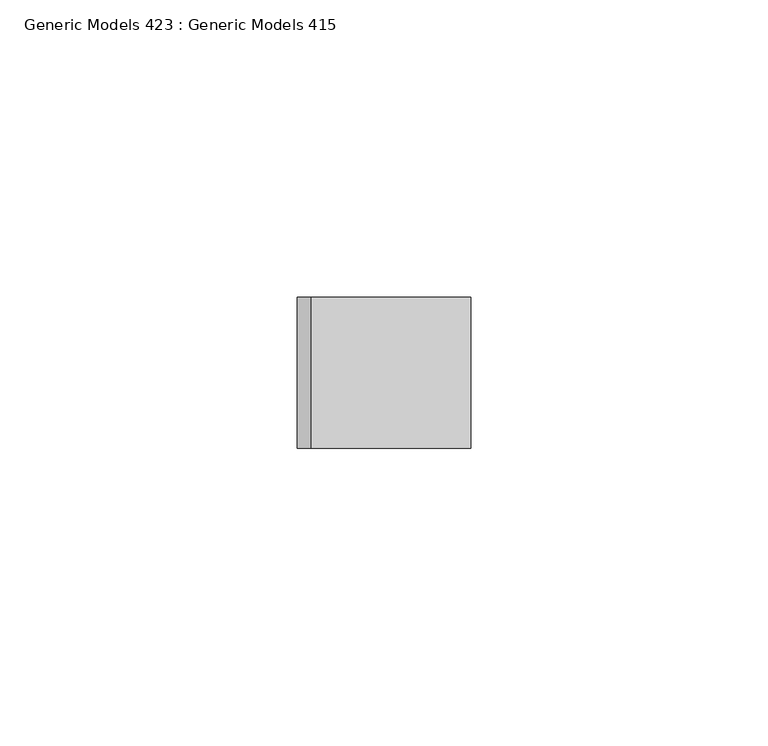
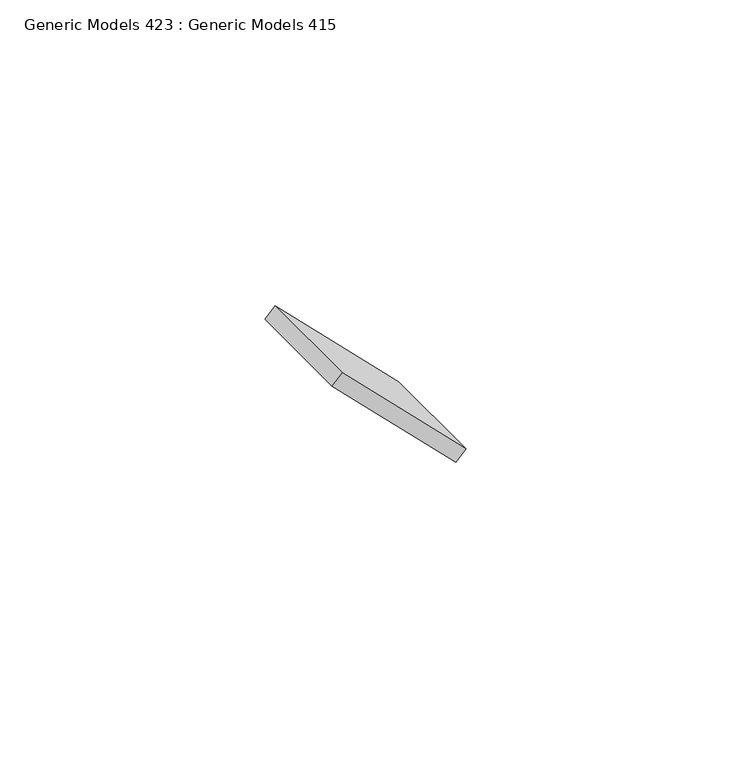
"""IFC4 building model written with IfcOpenShell, lengths in millimetres: proxy geometry, Generic Models 423 : Generic Models 415."""

from ifc_helpers import new_model, si_unit, frame, origin, place, context, project, spatial, polyline, outline, extrude, source, transform, mapped, element, save


def generic_models_423_generic_models_415_33f286a5(model_context):
    return source(origin(), model_context, "Body", "SweptSolid", [
        extrude(outline(polyline([(0.0, -38.1), (0.0, 0.0), (25.4, 0.0), (25.4, -38.1), (0.0, -38.1)])), frame((-6869.8996186, -4475.9863946, 128543.5002957), z_axis=(0.7071067811864907, 0.0, 0.7071067811866044), x_axis=(0.0, -1.0, 0.0)), (0.0, 0.0, 1.0), 3.175),
    ])


if __name__ == "__main__":
    model = new_model("IFC4")
    model_context = context("Model", 3, world=origin())
    ifc_project = project(units=[si_unit("LENGTHUNIT", "METRE", prefix="MILLI")], contexts=[model_context])
    site = spatial("IfcSite", under=ifc_project)
    building = spatial("IfcBuilding", under=site)
    placement = place(None, origin())
    generic_models_423_generic_models_415_shape = generic_models_423_generic_models_415_33f286a5(model_context)
    element("IfcBuildingElementProxy", 1, Name="Generic Models 423 : Generic Models 415", ObjectType="Generic Models 423 : Generic Models 415", at=placement, inside=building, context=model_context, shape_type="MappedRepresentation", body=[
        mapped(generic_models_423_generic_models_415_shape, transform((0.0, 0.0, 0.0), x_axis=(1.0, 0.0, 0.0), y_axis=(0.0, 1.0, 0.0), z_axis=(0.0, 0.0, 1.0))),
    ])
    save(model, "model.ifc")

# Revit data of these elements
# Element 1 (IfcBuildingElementProxy, "Generic Models 423 : Generic Models 415")
#   Materials on its faces: "_WELDED STEEL TABS FOR LOUVER ATTACHMENT"
# Materials
#   "_WELDED STEEL TABS FOR LOUVER ATTACHMENT": class "Metal", colour RGB 199 199 199, transparency 0, Description = "Structural steel 50ksi", Cost = 0
